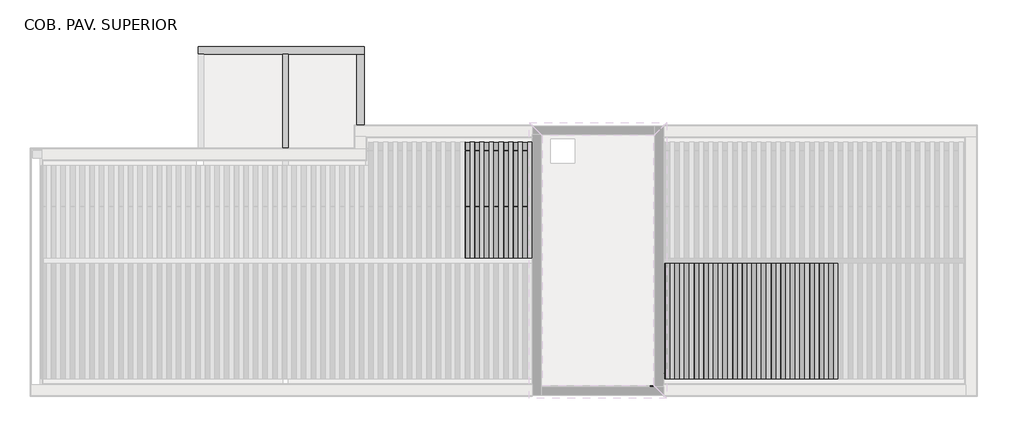
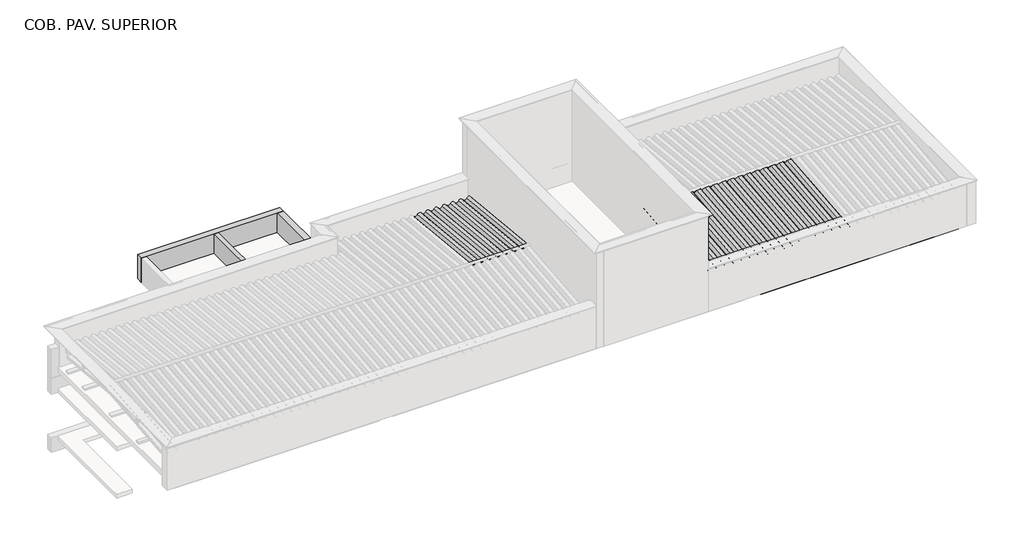
# One storey, part 5 of 7: 41 beams, 9 columns.
"""IFC4 building model written with IfcOpenShell, lengths in millimetres."""

import ifcopenshell
import ifcopenshell.guid

model = None  # the IFC model being written
_history = None  # IfcOwnerHistory: only IFC2X3 demands one
_inside = {}  # id of a spatial element -> (the spatial element, [elements in it])
_under = {}  # id of a project, library or spatial element -> (it, [spatial elements below it])
_declared = {}  # id of a project -> (the project, [libraries it declares])
_typed = {}  # id of a type object -> (the type object, [elements of that type])
_made_of = {}  # id of a material, layer set ... -> (it, [elements and type objects made of it])


def new_model(schema):
    """Start an empty IFC model of exactly this schema.

    Asked for "IFC4X3", IfcOpenShell would pick the latest addendum, in which some entities
    have other attributes; the version numbers below select the first issue.
    IFC2X3 requires an IfcOwnerHistory on every rooted entity: one is made here for all.
    """
    global model, _history
    if schema == "IFC4X3":
        model = ifcopenshell.file(schema_version=(4, 3, 0, 0))
    else:
        model = ifcopenshell.file(schema=schema)
    _inside.clear()
    _under.clear()
    _declared.clear()
    _typed.clear()
    _made_of.clear()
    _history = None
    if model.schema == "IFC2X3":
        org = make("IfcOrganization", Name="unknown")
        user = make(
            "IfcPersonAndOrganization",
            ThePerson=make("IfcPerson", FamilyName="unknown"),
            TheOrganization=org,
        )
        app = make(
            "IfcApplication",
            ApplicationDeveloper=org,
            Version="unknown",
            ApplicationFullName="unknown",
            ApplicationIdentifier="unknown",
        )
        _history = make(
            "IfcOwnerHistory",
            OwningUser=user,
            OwningApplication=app,
            ChangeAction="ADDED",
            CreationDate=0,
        )
    return model


def make(cls, **values):
    """One entity of the class cls with the attributes given. An attribute that is None is left unset."""
    return model.create_entity(
        cls, **{name: value for name, value in values.items() if value is not None}
    )


def rooted(cls, **values):
    """An entity with a GlobalId (a new one), such as an element, a storey or a relation."""
    return make(cls, GlobalId=ifcopenshell.guid.new(), OwnerHistory=_history, **values)


def si_unit(unit_type, name, prefix=None):
    """IfcSIUnit, for example si_unit("LENGTHUNIT", "METRE", prefix="MILLI")."""
    return make("IfcSIUnit", UnitType=unit_type, Prefix=prefix, Name=name)


def assignment(units):
    """IfcUnitAssignment: the units of a project."""
    return None if units is None else make("IfcUnitAssignment", Units=units)


def point(xyz):
    """IfcCartesianPoint."""
    return None if xyz is None else make("IfcCartesianPoint", Coordinates=xyz)


def direction(xyz):
    """IfcDirection."""
    return None if xyz is None else make("IfcDirection", DirectionRatios=xyz)


def frame(location, z_axis=None, x_axis=None):
    """IfcAxis2Placement3D, a coordinate frame: its origin and axes. An axis left out is left unset."""
    return make(
        "IfcAxis2Placement3D",
        Location=point(location),
        Axis=direction(z_axis),
        RefDirection=direction(x_axis),
    )


def frame_2d(location, x_axis=None):
    """IfcAxis2Placement2D, a coordinate frame in the plane: its origin and x axis."""
    return make(
        "IfcAxis2Placement2D", Location=point(location), RefDirection=direction(x_axis)
    )


def origin():
    """The frame at (0, 0, 0) with its axes left unset."""
    return frame((0.0, 0.0, 0.0))


def place(relative_to, where):
    """IfcLocalPlacement: puts the frame where relative to a parent placement (None: the world)."""
    return make(
        "IfcLocalPlacement", PlacementRelTo=relative_to, RelativePlacement=where
    )


def context(
    kind, dimensions, precision=None, world=None, true_north=None, identifier=None
):
    """IfcGeometricRepresentationContext, for example the 3D "Model" context."""
    return make(
        "IfcGeometricRepresentationContext",
        ContextIdentifier=identifier,
        ContextType=kind,
        CoordinateSpaceDimension=dimensions,
        Precision=precision,
        WorldCoordinateSystem=world,
        TrueNorth=true_north,
    )


def project(units=None, contexts=None):
    """IfcProject with its units and contexts."""
    return rooted(
        "IfcProject",
        Name="project",
        RepresentationContexts=contexts,
        UnitsInContext=assignment(units),
    )


def spatial(cls, under=None, at=None, **own):
    """A site, building, storey or space (cls), placed at a placement, below another one or the project."""
    s = rooted(cls, ObjectPlacement=at, **own)
    if under is not None:
        _under.setdefault(under.id(), (under, []))[1].append(s)
    return s


def polyline(points):
    """IfcPolyline through the points."""
    return make("IfcPolyline", Points=[point(p) for p in points])


def circle_curve(where, radius):
    """IfcCircle in the frame where."""
    return make("IfcCircle", Position=where, Radius=radius)


def trimmed(basis, trim1, trim2, sense, master):
    """IfcTrimmedCurve: the piece of a basis curve between two trims."""
    return make(
        "IfcTrimmedCurve",
        BasisCurve=basis,
        Trim1=trim1,
        Trim2=trim2,
        SenseAgreement=sense,
        MasterRepresentation=master,
    )


def segment(curve, same_sense, transition):
    """IfcCompositeCurveSegment."""
    return make(
        "IfcCompositeCurveSegment",
        Transition=transition,
        SameSense=same_sense,
        ParentCurve=curve,
    )


def composite_curve(segments, self_intersect=None):
    """IfcCompositeCurve: segments joined end to end."""
    return make("IfcCompositeCurve", Segments=segments, SelfIntersect=self_intersect)


def outline(outer, holes=None, kind="AREA"):
    """IfcArbitraryClosedProfileDef: a profile drawn as a closed curve; with holes, ...WithVoids."""
    if holes is None:
        return make("IfcArbitraryClosedProfileDef", ProfileType=kind, OuterCurve=outer)
    return make(
        "IfcArbitraryProfileDefWithVoids",
        ProfileType=kind,
        OuterCurve=outer,
        InnerCurves=holes,
    )


def extrude(swept, where, along, depth):
    """IfcExtrudedAreaSolid: the profile swept, set in the frame where, extruded along a direction by depth."""
    return make(
        "IfcExtrudedAreaSolid",
        SweptArea=swept,
        Position=where,
        ExtrudedDirection=direction(along),
        Depth=depth,
    )


def faces_of(points, faces, orient=None, outer=None):
    """IfcFace entities. A face is a list of loops; a loop is a list of indices into points, from 0.

    orient and outer hold one flag for each loop. By default every Orientation is true, the
    first loop of a face is its IfcFaceOuterBound and the others are IfcFaceBound.
    """
    made = []
    for i, loops in enumerate(faces):
        bounds = []
        for j, loop in enumerate(loops):
            is_outer = j == 0 if outer is None else outer[i][j]
            bounds.append(
                make(
                    "IfcFaceOuterBound" if is_outer else "IfcFaceBound",
                    Bound=make("IfcPolyLoop", Polygon=[points[k] for k in loop]),
                    Orientation=True if orient is None else orient[i][j],
                )
            )
        made.append(make("IfcFace", Bounds=bounds))
    return made


def faceted_brep(points, faces, orient=None, outer=None, voids=None):
    """IfcFacetedBrep: a solid bounded by flat faces; with voids (closed shells), ...WithVoids."""
    shared = [point(p) for p in points]
    hull = make("IfcClosedShell", CfsFaces=faces_of(shared, faces, orient, outer))
    if voids is None:
        return make("IfcFacetedBrep", Outer=hull)
    return make(
        "IfcFacetedBrepWithVoids",
        Outer=hull,
        Voids=[
            make(cls, CfsFaces=faces_of(shared, fs, o, b)) for cls, fs, o, b in voids
        ],
    )


def shape(context_of_items, identifier, shape_type, items):
    """IfcShapeRepresentation: the items that make up one representation, for example the "Body"."""
    return make(
        "IfcShapeRepresentation",
        ContextOfItems=context_of_items,
        RepresentationIdentifier=identifier,
        RepresentationType=shape_type,
        Items=items,
    )


def source(mapping_origin, context_of_items, identifier, shape_type, items):
    """IfcRepresentationMap: a shape defined once, which mapped items show again and again."""
    return make(
        "IfcRepresentationMap",
        MappingOrigin=mapping_origin,
        MappedRepresentation=shape(context_of_items, identifier, shape_type, items),
    )


def transform(
    local_origin,
    x_axis=None,
    y_axis=None,
    z_axis=None,
    scale=None,
    scale2=None,
    scale3=None,
    uniform=True,
):
    """IfcCartesianTransformationOperator3D, or its non-uniform kind. x_axis, y_axis, z_axis: its Axis1, 2, 3."""
    if uniform:
        return make(
            "IfcCartesianTransformationOperator3D",
            Axis1=direction(x_axis),
            Axis2=direction(y_axis),
            LocalOrigin=point(local_origin),
            Scale=scale,
            Axis3=direction(z_axis),
        )
    return make(
        "IfcCartesianTransformationOperator3DnonUniform",
        Axis1=direction(x_axis),
        Axis2=direction(y_axis),
        LocalOrigin=point(local_origin),
        Scale=scale,
        Axis3=direction(z_axis),
        Scale2=scale2,
        Scale3=scale3,
    )


def mapped(mapping_source, mapping_target):
    """IfcMappedItem: shows the shape of a source again, moved by a transform."""
    return make(
        "IfcMappedItem", MappingSource=mapping_source, MappingTarget=mapping_target
    )


def made_of(thing, what):
    """Note that an element or type object is made of a material, layer set ...; save() writes the relation."""
    if what is not None:
        _made_of.setdefault(what.id(), (what, []))[1].append(thing)
    return thing


def element(
    cls,
    number,
    at=None,
    inside=None,
    cuts=None,
    type_object=None,
    material=None,
    context=None,
    identifier="Body",
    shape_type=None,
    held_by="IfcProductDefinitionShape",
    body=None,
    shapes=None,
    **own,
):
    """One element of the class cls, such as IfcWall. Its Tag is "e" and its number.

    at: its placement. inside: the storey or other place that contains it. cuts: it is an
    opening in that element (IfcRelVoidsElement). A single representation is given by context,
    identifier, shape_type and body (its items); several are given by shapes. held_by: the class
    of the entity that holds the representations. save() writes the other relations.
    """
    e = rooted(cls, Tag="e%d" % number, ObjectPlacement=at, **own)
    if body is not None:
        shapes = [shape(context, identifier, shape_type, body)]
    if shapes is not None:
        e.Representation = make(held_by, Representations=shapes)
    if inside is not None:
        _inside.setdefault(inside.id(), (inside, []))[1].append(e)
    if cuts is not None:
        rooted(
            "IfcRelVoidsElement", RelatingBuildingElement=cuts, RelatedOpeningElement=e
        )
    if type_object is not None:
        _typed.setdefault(type_object.id(), (type_object, []))[1].append(e)
    return made_of(e, material)


def aggregate(whole, parts):
    """IfcRelAggregates: a whole, such as a stair, and the parts it consists of."""
    return rooted("IfcRelAggregates", RelatingObject=whole, RelatedObjects=parts)


def save(model, path):
    """Write the relations noted so far, then the file.

    IfcRelAggregates (storeys below a building ...), IfcRelContainedInSpatialStructure (elements
    in a storey), IfcRelDefinesByType, IfcRelAssociatesMaterial and IfcRelDeclares: one each for
    every whole, place, type object, material and project.
    """
    for whole, parts in _under.values():
        aggregate(whole, parts)
    for where, things in _inside.values():
        rooted(
            "IfcRelContainedInSpatialStructure",
            RelatedElements=things,
            RelatingStructure=where,
        )
    for kind, things in _typed.values():
        rooted("IfcRelDefinesByType", RelatedObjects=things, RelatingType=kind)
    for what, things in _made_of.values():
        rooted("IfcRelAssociatesMaterial", RelatedObjects=things, RelatingMaterial=what)
    for by, libraries in _declared.values():
        rooted("IfcRelDeclares", RelatingContext=by, RelatedDefinitions=libraries)
    model.write(path)


def column_d505325c(model_context):
    return source(origin(), model_context, "Body", "SweptSolid", [
        extrude(outline(polyline([(30.0, 80.0), (30.0, -80.0), (-30.0, -80.0), (-30.0, 80.0), (30.0, 80.0)])), frame((0.0, 0.0, 6710.0), z_axis=(0.0, 0.0, 1.0), x_axis=(1.0, 0.0, 0.0)), (0.0, 0.0, 1.0), 750.0),
    ])


def column_4db371bd(model_context):
    return source(origin(), model_context, "Body", "SweptSolid", [
        extrude(outline(polyline([(30.0, 80.0), (30.0, -80.0), (-30.0, -80.0), (-30.0, 80.0), (30.0, 80.0)])), frame((0.0, 0.0, 6710.0), z_axis=(0.0, 0.0, 1.0), x_axis=(1.0, 0.0, 0.0)), (0.0, 0.0, 1.0), 660.0),
    ])


def column_e8b88e91(model_context):
    return source(origin(), model_context, "Body", "SweptSolid", [
        extrude(outline(polyline([(30.0, 80.0), (30.0, -80.0), (-30.0, -80.0), (-30.0, 80.0), (30.0, 80.0)])), frame((0.0, 0.0, 6710.0), z_axis=(0.0, 0.0, 1.0), x_axis=(1.0, 0.0, 0.0)), (0.0, 0.0, 1.0), 515.0),
    ])


def column_d0cf395a(model_context):
    return source(origin(), model_context, "Body", "SweptSolid", [
        extrude(outline(polyline([(30.0, 80.0), (30.0, -80.0), (-30.0, -80.0), (-30.0, 80.0), (30.0, 80.0)])), frame((0.0, 0.0, 6710.0), z_axis=(0.0, 0.0, 1.0), x_axis=(1.0, 0.0, 0.0)), (0.0, 0.0, 1.0), 520.0),
    ])


model = new_model("IFC4")

# Units and contexts
model_context = context("Model", 3, world=origin())
ifc_project = project(units=[si_unit("LENGTHUNIT", "METRE", prefix="MILLI")], contexts=[model_context])

# Site, building, storey
site = spatial("IfcSite", under=ifc_project)
building = spatial("IfcBuilding", under=site)
storey = spatial("IfcBuildingStorey", under=building, Name="COB. PAV. SUPERIOR", Elevation=6650.0)

# Beams
placement = place(None, origin())
element("IfcBeam", 1, ObjectType="Madeira de lei : Berço 6x12cm", at=placement, inside=storey, context=model_context, shape_type="SweptSolid", body=[
    extrude(outline(polyline([(-679.281307, -7711.5607799), (-679.281307, -7831.5607799), (-2679.281307, -7831.5607799), (-2679.281307, -7711.5607799), (-679.281307, -7711.5607799)])), frame((0.0, 0.0, 6650.0), z_axis=(0.0, 0.0, 1.0), x_axis=(1.0, 0.0, 0.0)), (0.0, 0.0, 1.0), 60.0),
])
element("IfcBeam", 2, ObjectType="Madeira de lei : Berço 6x12cm", at=placement, inside=storey, context=model_context, shape_type="SweptSolid", body=[
    extrude(outline(polyline([(-244.281307, -7711.5607799), (-244.281307, -7831.5607799), (-679.281307, -7831.5607799), (-679.281307, -7711.5607799), (-244.281307, -7711.5607799)])), frame((0.0, 0.0, 6650.0), z_axis=(0.0, 0.0, 1.0), x_axis=(1.0, 0.0, 0.0)), (0.0, 0.0, 1.0), 60.0),
])
element("IfcBeam", 3, ObjectType="Madeira de lei : Berço 6x12cm", at=placement, inside=storey, context=model_context, shape_type="SweptSolid", body=[
    extrude(outline(polyline([(-679.2813076, -6319.8711004), (-679.2813076, -6439.8711004), (-2679.2813064, -6439.8711004), (-2679.2813064, -6319.8711004), (-679.2813076, -6319.8711004)])), frame((0.0, 0.0, 6650.0), z_axis=(0.0, 0.0, 1.0), x_axis=(1.0, 0.0, 0.0)), (0.0, 0.0, 1.0), 60.0),
])
element("IfcBeam", 4, ObjectType="Madeira de lei : Berço 6x12cm", at=placement, inside=storey, context=model_context, shape_type="SweptSolid", body=[
    extrude(outline(polyline([(-259.281307, -6319.8711004), (-259.281307, -6439.8711004), (-679.2813064, -6439.8711004), (-679.2813064, -6319.8711004), (-259.281307, -6319.8711004)])), frame((0.0, 0.0, 6650.0), z_axis=(0.0, 0.0, 1.0), x_axis=(1.0, 0.0, 0.0)), (0.0, 0.0, 1.0), 60.0),
])
element("IfcBeam", 5, ObjectType="Madeira de lei : Berço 6x12cm", at=placement, inside=storey, context=model_context, shape_type="SweptSolid", body=[
    extrude(outline(polyline([(5089.718693, -9101.268869), (5089.718693, -9221.268869), (3089.718693, -9221.268869), (3089.718693, -9101.268869), (5089.718693, -9101.268869)])), frame((0.0, 0.0, 6650.0), z_axis=(0.0, 0.0, 1.0), x_axis=(1.0, 0.0, 0.0)), (0.0, 0.0, 1.0), 60.0),
])
element("IfcBeam", 6, ObjectType="Madeira de lei : Berço 6x12cm", at=placement, inside=storey, context=model_context, shape_type="SweptSolid", body=[
    extrude(outline(polyline([(5089.718693, -10521.818869), (5089.718693, -10641.818869), (3089.718693, -10641.818869), (3089.718693, -10521.818869), (5089.718693, -10521.818869)])), frame((0.0, 0.0, 6650.0), z_axis=(0.0, 0.0, 1.0), x_axis=(1.0, 0.0, 0.0)), (0.0, 0.0, 1.0), 60.0),
])
element("IfcBeam", 7, ObjectType="Madeira de lei : Berço 6x12cm", at=placement, inside=storey, context=model_context, shape_type="SweptSolid", body=[
    extrude(outline(polyline([(7089.718693, -9101.268869), (7089.718693, -9221.268869), (5089.718693, -9221.268869), (5089.718693, -9101.268869), (7089.718693, -9101.268869)])), frame((0.0, 0.0, 6650.0), z_axis=(0.0, 0.0, 1.0), x_axis=(1.0, 0.0, 0.0)), (0.0, 0.0, 1.0), 60.0),
])
element("IfcBeam", 8, ObjectType="Madeira de lei : Berço 6x12cm", at=placement, inside=storey, context=model_context, shape_type="SweptSolid", body=[
    extrude(outline(polyline([(7089.718693, -10521.818869), (7089.718693, -10641.818869), (5089.718693, -10641.818869), (5089.718693, -10521.818869), (7089.718693, -10521.818869)])), frame((0.0, 0.0, 6650.0), z_axis=(0.0, 0.0, 1.0), x_axis=(1.0, 0.0, 0.0)), (0.0, 0.0, 1.0), 60.0),
])
element("IfcBeam", 9, ObjectType="Madeira de lei : Berço 6x12cm", at=placement, inside=storey, context=model_context, shape_type="SweptSolid", body=[
    extrude(outline(polyline([(-270.281307, -4899.3026908), (-270.281307, -5019.3026908), (-2270.2813064, -5019.3026908), (-2270.2813064, -4899.3026908), (-270.281307, -4899.3026908)])), frame((0.0, 0.0, 6650.0), z_axis=(0.0, 0.0, 1.0), x_axis=(1.0, 0.0, 0.0)), (0.0, 0.0, 1.0), 60.0),
])
element("IfcBeam", 10, ObjectType="Madeira de lei : Berço 6x12cm", at=placement, inside=storey, context=model_context, shape_type="SweptSolid", body=[
    extrude(outline(polyline([(-2270.2813076, -4899.3026908), (-2270.2813076, -5019.3026908), (-4270.281307, -5019.3026908), (-4270.281307, -4899.3026908), (-2270.2813076, -4899.3026908)])), frame((0.0, 0.0, 6650.0), z_axis=(0.0, 0.0, 1.0), x_axis=(1.0, 0.0, 0.0)), (0.0, 0.0, 1.0), 60.0),
])
element("IfcBeam", 11, ObjectType="TQS - Viga retangular : 14.0 x 76.0", at=placement, inside=storey, context=model_context, shape_type="Brep", body=[
    faceted_brep([(-6580.281307, -4975.5699847, 7050.0), (-6440.281307, -4975.5699847, 7050.0), (-6440.281307, -2515.5699847, 7050.0), (-6580.281307, -2515.5699847, 7050.0), (-6440.281307, -4975.5699847, 6450.0), (-6440.281307, -4975.5699847, 6290.0), (-6440.281307, -2515.5699847, 6290.0), (-6440.281307, -2515.5699847, 6450.0), (-6580.281307, -4975.5699847, 6290.0), (-6580.281307, -2515.5699847, 6290.0), (-6580.281307, -4975.5699847, 6450.0), (-6580.281307, -2515.5699847, 6450.0)], [[[0, 1, 2, 3]], [[1, 4, 5, 6, 7, 2]], [[5, 8, 9, 6]], [[8, 10, 0, 3, 11, 9]], [[0, 10, 8, 5, 4, 1]], [[3, 2, 7, 6, 9, 11]]]),
])
element("IfcBeam", 12, ObjectType="TQS - Viga retangular : 19.0 x 60.0", at=placement, inside=storey, context=model_context, shape_type="Brep", body=[
    faceted_brep([(-12.281307, -4775.5699847, 7050.0), (-202.281307, -4775.5699847, 7050.0), (-202.281307, -10953.5699847, 7050.0), (-12.281307, -10953.5699847, 7050.0), (-12.281307, -4775.5699847, 6450.0), (-12.281307, -10953.5699847, 6650.0), (-12.281307, -10953.5699847, 6450.0), (-202.281307, -4775.5699847, 6450.0), (-202.281307, -10953.5699847, 6450.0), (-202.281307, -10953.5699847, 6650.0)], [[[0, 1, 2, 3]], [[4, 0, 3, 5, 6]], [[7, 4, 6, 8]], [[1, 7, 8, 9, 2]], [[1, 0, 4, 7]], [[2, 9, 8, 6, 5, 3]]]),
])
element("IfcBeam", 13, ObjectType="TQS - Viga retangular : 19.0 x 76.0", at=placement, inside=storey, context=model_context, shape_type="Brep", body=[
    faceted_brep([(-8730.281307, -2325.5699847, 7050.0), (-8730.281307, -2515.5699847, 7050.0), (-8590.281307, -2515.5699847, 7050.0), (-6580.281307, -2515.5699847, 7050.0), (-6440.281307, -2515.5699847, 7050.0), (-4702.281307, -2515.5699847, 7050.0), (-4512.281307, -2515.5699847, 7050.0), (-4512.281307, -2325.5699847, 7050.0), (-8730.281307, -2515.5699847, 6290.0), (-8590.281307, -2515.5699847, 6290.0), (-6580.281307, -2515.5699847, 6290.0), (-6440.281307, -2515.5699847, 6290.0), (-4702.281307, -2515.5699847, 6290.0), (-4512.281307, -2515.5699847, 6290.0), (-8730.281307, -2325.5699847, 6290.0), (-4512.281307, -2325.5699847, 6290.0)], [[[0, 1, 2, 3, 4, 5, 6, 7]], [[1, 8, 9, 10, 11, 12, 13, 6, 5, 4, 3, 2]], [[8, 14, 15, 13, 12, 11, 10, 9]], [[14, 0, 7, 15]], [[1, 0, 14, 8]], [[7, 6, 13, 15]]]),
])
element("IfcBeam", 14, ObjectType="TQS - Viga retangular : 19.0 x 76.0", at=placement, inside=storey, context=model_context, shape_type="Brep", body=[
    faceted_brep([(-4512.281307, -2515.5699847, 7050.0), (-4702.281307, -2515.5699847, 7050.0), (-4702.281307, -4375.5699847, 7050.0), (-4512.281307, -4375.5699847, 7050.0), (-4512.281307, -2515.5699847, 6290.0), (-4512.281307, -4375.5699847, 6290.0), (-4702.281307, -2515.5699847, 6290.0), (-4702.281307, -4375.5699847, 6290.0), (-4702.281307, -2515.5699847, 6450.0)], [[[0, 1, 2, 3]], [[4, 0, 3, 5]], [[6, 4, 5, 7]], [[1, 8, 6, 7, 2]], [[1, 0, 4, 6, 8]], [[3, 2, 7, 5]]]),
])
element("IfcBeam", 15, ObjectType="TQS - Viga retangular : 19.0 x 80.0", at=placement, inside=storey, context=model_context, shape_type="SweptSolid", body=[
    extrude(outline(polyline([(10537.718693, -10953.5699847), (10537.718693, -11143.5699847), (4678.718693, -11143.5699847), (4678.718693, -10953.5699847), (10537.718693, -10953.5699847)])), frame((0.0, 0.0, 6450.0), z_axis=(0.0, 0.0, 1.0), x_axis=(1.0, 0.0, 0.0)), (0.0, 0.0, 1.0), 800.0),
])
element("IfcBeam", 16, ObjectType="TQS - Viga retangular : 19.0 x 80.0", at=placement, inside=storey, context=model_context, shape_type="Brep", body=[
    faceted_brep([(-4142.481307, -4375.5699847, 7250.0), (-4142.481307, -4565.5699847, 7250.0), (-202.281307, -4565.5699847, 7250.0), (-202.281307, -4375.5699847, 7250.0), (-4142.481307, -4565.5699847, 6450.0), (-202.281307, -4565.5699847, 6450.0), (-202.281307, -4565.5699847, 6650.0), (-4142.481307, -4375.5699847, 6450.0), (-202.281307, -4375.5699847, 6450.0)], [[[0, 1, 2, 3]], [[1, 4, 5, 6, 2]], [[4, 7, 8, 5]], [[7, 0, 3, 8]], [[1, 0, 7, 4]], [[3, 2, 6, 5, 8]]]),
    faceted_brep([(-4442.481307, -4375.5699847, 7250.0), (-4442.481307, -4565.5699847, 7250.0), (-4442.481307, -4565.5699847, 6450.0), (-4442.481307, -4375.5699847, 6450.0), (-4512.281307, -4375.5699847, 7250.0), (-4512.281307, -4565.5699847, 7250.0), (-4512.281307, -4565.5699847, 6650.0), (-4512.281307, -4565.5699847, 6450.0), (-4512.281307, -4375.5699847, 6450.0)], [[[0, 1, 2, 3]], [[1, 0, 4, 5]], [[2, 1, 5, 6, 7]], [[3, 2, 7, 8]], [[0, 3, 8, 4]], [[5, 4, 8, 7, 6]]]),
])
element("IfcBeam", 17, ObjectType="Telha Ondulada : Fibrocimento", at=placement, inside=storey, context=model_context, shape_type="SweptSolid", body=[
    extrude(outline(composite_curve([segment(trimmed(circle_curve(frame_2d((0.0, 66.7939461)), 66.7939461), [point((29.3501489, 6.7939461))], [point((29.3501489, 126.7939461))], True, "CARTESIAN"), True, "CONTINUOUS"), segment(polyline([(29.3501489, 126.7939461), (31.5472154, 131.2853711)]), True, "CONTINUOUS"), segment(trimmed(circle_curve(frame_2d((0.0, 66.7939461)), 71.7939461), [point((31.5472154, 131.2853711))], [point((31.5472154, 2.3025211))], False, "CARTESIAN"), True, "CONTINUOUS"), segment(trimmed(circle_curve(frame_2d((58.7002978, -53.2060539)), 61.7939461), [point((31.5472154, 2.3025211))], [point((31.5472154, -108.7146289))], True, "CARTESIAN"), True, "CONTINUOUS"), segment(polyline([(31.5472154, -108.7146289), (29.3501489, -113.2060539)]), True, "CONTINUOUS"), segment(trimmed(circle_curve(frame_2d((58.7002978, -53.2060539)), 66.7939461), [point((29.3501489, -113.2060539))], [point((29.3501489, 6.7939461))], False, "CARTESIAN"), True, "CONTINUOUS")], self_intersect=False)), frame((3256.1156257, -10781.9594023, 7394.5315886), z_axis=(0.0, 0.9950371902099894, 0.09950371902099751), x_axis=(0.0, 0.09950371902099751, -0.9950371902099894)), (0.0, 0.0, 1.0), 3017.2387654),
])
element("IfcBeam", 18, ObjectType="Telha Ondulada : Fibrocimento", at=placement, inside=storey, context=model_context, shape_type="SweptSolid", body=[
    extrude(outline(composite_curve([segment(trimmed(circle_curve(frame_2d((0.0, 66.7939461)), 66.7939461), [point((29.3501489, 6.7939461))], [point((29.3501489, 126.7939461))], True, "CARTESIAN"), True, "CONTINUOUS"), segment(polyline([(29.3501489, 126.7939461), (31.5472154, 131.2853711)]), True, "CONTINUOUS"), segment(trimmed(circle_curve(frame_2d((0.0, 66.7939461)), 71.7939461), [point((31.5472154, 131.2853711))], [point((31.5472154, 2.3025211))], False, "CARTESIAN"), True, "CONTINUOUS"), segment(trimmed(circle_curve(frame_2d((58.7002978, -53.2060539)), 61.7939461), [point((31.5472154, 2.3025211))], [point((31.5472154, -108.7146289))], True, "CARTESIAN"), True, "CONTINUOUS"), segment(polyline([(31.5472154, -108.7146289), (29.3501489, -113.2060539)]), True, "CONTINUOUS"), segment(trimmed(circle_curve(frame_2d((58.7002978, -53.2060539)), 66.7939461), [point((29.3501489, -113.2060539))], [point((29.3501489, 6.7939461))], False, "CARTESIAN"), True, "CONTINUOUS")], self_intersect=False)), frame((3500.6156257, -10781.9594023, 7394.5315886), z_axis=(0.0, 0.9950371902099894, 0.09950371902099751), x_axis=(0.0, 0.09950371902099751, -0.9950371902099894)), (0.0, 0.0, 1.0), 3017.2387654),
])
element("IfcBeam", 19, ObjectType="Telha Ondulada : Fibrocimento", at=placement, inside=storey, context=model_context, shape_type="SweptSolid", body=[
    extrude(outline(composite_curve([segment(trimmed(circle_curve(frame_2d((0.0, 66.7939461)), 66.7939461), [point((29.3501489, 6.7939461))], [point((29.3501489, 126.7939461))], True, "CARTESIAN"), True, "CONTINUOUS"), segment(polyline([(29.3501489, 126.7939461), (31.5472154, 131.2853711)]), True, "CONTINUOUS"), segment(trimmed(circle_curve(frame_2d((0.0, 66.7939461)), 71.7939461), [point((31.5472154, 131.2853711))], [point((31.5472154, 2.3025211))], False, "CARTESIAN"), True, "CONTINUOUS"), segment(trimmed(circle_curve(frame_2d((58.7002978, -53.2060539)), 61.7939461), [point((31.5472154, 2.3025211))], [point((31.5472154, -108.7146289))], True, "CARTESIAN"), True, "CONTINUOUS"), segment(polyline([(31.5472154, -108.7146289), (29.3501489, -113.2060539)]), True, "CONTINUOUS"), segment(trimmed(circle_curve(frame_2d((58.7002978, -53.2060539)), 66.7939461), [point((29.3501489, -113.2060539))], [point((29.3501489, 6.7939461))], False, "CARTESIAN"), True, "CONTINUOUS")], self_intersect=False)), frame((3745.1156257, -10781.9594023, 7394.5315886), z_axis=(0.0, 0.9950371902099894, 0.09950371902099751), x_axis=(0.0, 0.09950371902099751, -0.9950371902099894)), (0.0, 0.0, 1.0), 3017.2387654),
])
element("IfcBeam", 20, ObjectType="Telha Ondulada : Fibrocimento", at=placement, inside=storey, context=model_context, shape_type="SweptSolid", body=[
    extrude(outline(composite_curve([segment(trimmed(circle_curve(frame_2d((0.0, 66.7939461)), 66.7939461), [point((29.3501489, 6.7939461))], [point((29.3501489, 126.7939461))], True, "CARTESIAN"), True, "CONTINUOUS"), segment(polyline([(29.3501489, 126.7939461), (31.5472154, 131.2853711)]), True, "CONTINUOUS"), segment(trimmed(circle_curve(frame_2d((0.0, 66.7939461)), 71.7939461), [point((31.5472154, 131.2853711))], [point((31.5472154, 2.3025211))], False, "CARTESIAN"), True, "CONTINUOUS"), segment(trimmed(circle_curve(frame_2d((58.7002978, -53.2060539)), 61.7939461), [point((31.5472154, 2.3025211))], [point((31.5472154, -108.7146289))], True, "CARTESIAN"), True, "CONTINUOUS"), segment(polyline([(31.5472154, -108.7146289), (29.3501489, -113.2060539)]), True, "CONTINUOUS"), segment(trimmed(circle_curve(frame_2d((58.7002978, -53.2060539)), 66.7939461), [point((29.3501489, -113.2060539))], [point((29.3501489, 6.7939461))], False, "CARTESIAN"), True, "CONTINUOUS")], self_intersect=False)), frame((3989.6156257, -10781.9594023, 7394.5315886), z_axis=(0.0, 0.9950371902099894, 0.09950371902099747), x_axis=(0.0, 0.09950371902099747, -0.9950371902099894)), (0.0, 0.0, 1.0), 3017.2387654),
])
element("IfcBeam", 21, ObjectType="Telha Ondulada : Fibrocimento", at=placement, inside=storey, context=model_context, shape_type="SweptSolid", body=[
    extrude(outline(composite_curve([segment(trimmed(circle_curve(frame_2d((0.0, 66.7939461)), 66.7939461), [point((29.3501489, 6.7939461))], [point((29.3501489, 126.7939461))], True, "CARTESIAN"), True, "CONTINUOUS"), segment(polyline([(29.3501489, 126.7939461), (31.5472154, 131.2853711)]), True, "CONTINUOUS"), segment(trimmed(circle_curve(frame_2d((0.0, 66.7939461)), 71.7939461), [point((31.5472154, 131.2853711))], [point((31.5472154, 2.3025211))], False, "CARTESIAN"), True, "CONTINUOUS"), segment(trimmed(circle_curve(frame_2d((58.7002978, -53.2060539)), 61.7939461), [point((31.5472154, 2.3025211))], [point((31.5472154, -108.7146289))], True, "CARTESIAN"), True, "CONTINUOUS"), segment(polyline([(31.5472154, -108.7146289), (29.3501489, -113.2060539)]), True, "CONTINUOUS"), segment(trimmed(circle_curve(frame_2d((58.7002978, -53.2060539)), 66.7939461), [point((29.3501489, -113.2060539))], [point((29.3501489, 6.7939461))], False, "CARTESIAN"), True, "CONTINUOUS")], self_intersect=False)), frame((4234.1156257, -10781.9594023, 7394.5315886), z_axis=(0.0, 0.9950371902099894, 0.09950371902099747), x_axis=(0.0, 0.09950371902099747, -0.9950371902099894)), (0.0, 0.0, 1.0), 3017.2387654),
])
element("IfcBeam", 22, ObjectType="Telha Ondulada : Fibrocimento", at=placement, inside=storey, context=model_context, shape_type="SweptSolid", body=[
    extrude(outline(composite_curve([segment(trimmed(circle_curve(frame_2d((0.0, 66.7939461)), 66.7939461), [point((29.3501489, 6.7939461))], [point((29.3501489, 126.7939461))], True, "CARTESIAN"), True, "CONTINUOUS"), segment(polyline([(29.3501489, 126.7939461), (31.5472154, 131.2853711)]), True, "CONTINUOUS"), segment(trimmed(circle_curve(frame_2d((0.0, 66.7939461)), 71.7939461), [point((31.5472154, 131.2853711))], [point((31.5472154, 2.3025211))], False, "CARTESIAN"), True, "CONTINUOUS"), segment(trimmed(circle_curve(frame_2d((58.7002978, -53.2060539)), 61.7939461), [point((31.5472154, 2.3025211))], [point((31.5472154, -108.7146289))], True, "CARTESIAN"), True, "CONTINUOUS"), segment(polyline([(31.5472154, -108.7146289), (29.3501489, -113.2060539)]), True, "CONTINUOUS"), segment(trimmed(circle_curve(frame_2d((58.7002978, -53.2060539)), 66.7939461), [point((29.3501489, -113.2060539))], [point((29.3501489, 6.7939461))], False, "CARTESIAN"), True, "CONTINUOUS")], self_intersect=False)), frame((4478.6156257, -10781.9594023, 7394.5315886), z_axis=(0.0, 0.9950371902099894, 0.09950371902099744), x_axis=(0.0, 0.09950371902099744, -0.9950371902099894)), (0.0, 0.0, 1.0), 3017.2387654),
])
element("IfcBeam", 23, ObjectType="Telha Ondulada : Fibrocimento", at=placement, inside=storey, context=model_context, shape_type="SweptSolid", body=[
    extrude(outline(composite_curve([segment(trimmed(circle_curve(frame_2d((0.0, 66.7939461)), 66.7939461), [point((29.3501489, 6.7939461))], [point((29.3501489, 126.7939461))], True, "CARTESIAN"), True, "CONTINUOUS"), segment(polyline([(29.3501489, 126.7939461), (31.5472154, 131.2853711)]), True, "CONTINUOUS"), segment(trimmed(circle_curve(frame_2d((0.0, 66.7939461)), 71.7939461), [point((31.5472154, 131.2853711))], [point((31.5472154, 2.3025211))], False, "CARTESIAN"), True, "CONTINUOUS"), segment(trimmed(circle_curve(frame_2d((58.7002978, -53.2060539)), 61.7939461), [point((31.5472154, 2.3025211))], [point((31.5472154, -108.7146289))], True, "CARTESIAN"), True, "CONTINUOUS"), segment(polyline([(31.5472154, -108.7146289), (29.3501489, -113.2060539)]), True, "CONTINUOUS"), segment(trimmed(circle_curve(frame_2d((58.7002978, -53.2060539)), 66.7939461), [point((29.3501489, -113.2060539))], [point((29.3501489, 6.7939461))], False, "CARTESIAN"), True, "CONTINUOUS")], self_intersect=False)), frame((4723.1156257, -10781.9594023, 7394.5315886), z_axis=(0.0, 0.9950371902099894, 0.09950371902099751), x_axis=(0.0, 0.09950371902099751, -0.9950371902099894)), (0.0, 0.0, 1.0), 3017.2387654),
])
element("IfcBeam", 24, ObjectType="Telha Ondulada : Fibrocimento", at=placement, inside=storey, context=model_context, shape_type="SweptSolid", body=[
    extrude(outline(composite_curve([segment(trimmed(circle_curve(frame_2d((0.0, 66.7939461)), 66.7939461), [point((29.3501489, 6.7939461))], [point((29.3501489, 126.7939461))], True, "CARTESIAN"), True, "CONTINUOUS"), segment(polyline([(29.3501489, 126.7939461), (31.5472154, 131.2853711)]), True, "CONTINUOUS"), segment(trimmed(circle_curve(frame_2d((0.0, 66.7939461)), 71.7939461), [point((31.5472154, 131.2853711))], [point((31.5472154, 2.3025211))], False, "CARTESIAN"), True, "CONTINUOUS"), segment(trimmed(circle_curve(frame_2d((58.7002978, -53.2060539)), 61.7939461), [point((31.5472154, 2.3025211))], [point((31.5472154, -108.7146289))], True, "CARTESIAN"), True, "CONTINUOUS"), segment(polyline([(31.5472154, -108.7146289), (29.3501489, -113.2060539)]), True, "CONTINUOUS"), segment(trimmed(circle_curve(frame_2d((58.7002978, -53.2060539)), 66.7939461), [point((29.3501489, -113.2060539))], [point((29.3501489, 6.7939461))], False, "CARTESIAN"), True, "CONTINUOUS")], self_intersect=False)), frame((4967.6156257, -10781.9594023, 7394.5315886), z_axis=(0.0, 0.9950371902099894, 0.09950371902099751), x_axis=(0.0, 0.09950371902099751, -0.9950371902099894)), (0.0, 0.0, 1.0), 3017.2387654),
])
element("IfcBeam", 25, ObjectType="Telha Ondulada : Fibrocimento", at=placement, inside=storey, context=model_context, shape_type="SweptSolid", body=[
    extrude(outline(composite_curve([segment(trimmed(circle_curve(frame_2d((0.0, 66.7939461)), 66.7939461), [point((29.3501489, 6.7939461))], [point((29.3501489, 126.7939461))], True, "CARTESIAN"), True, "CONTINUOUS"), segment(polyline([(29.3501489, 126.7939461), (31.5472154, 131.2853711)]), True, "CONTINUOUS"), segment(trimmed(circle_curve(frame_2d((0.0, 66.7939461)), 71.7939461), [point((31.5472154, 131.2853711))], [point((31.5472154, 2.3025211))], False, "CARTESIAN"), True, "CONTINUOUS"), segment(trimmed(circle_curve(frame_2d((58.7002978, -53.2060539)), 61.7939461), [point((31.5472154, 2.3025211))], [point((31.5472154, -108.7146289))], True, "CARTESIAN"), True, "CONTINUOUS"), segment(polyline([(31.5472154, -108.7146289), (29.3501489, -113.2060539)]), True, "CONTINUOUS"), segment(trimmed(circle_curve(frame_2d((58.7002978, -53.2060539)), 66.7939461), [point((29.3501489, -113.2060539))], [point((29.3501489, 6.7939461))], False, "CARTESIAN"), True, "CONTINUOUS")], self_intersect=False)), frame((5212.1156257, -10781.9594023, 7394.5315886), z_axis=(0.0, 0.9950371902099894, 0.09950371902099751), x_axis=(0.0, 0.09950371902099751, -0.9950371902099894)), (0.0, 0.0, 1.0), 3017.2387654),
])
element("IfcBeam", 26, ObjectType="Telha Ondulada : Fibrocimento", at=placement, inside=storey, context=model_context, shape_type="SweptSolid", body=[
    extrude(outline(composite_curve([segment(trimmed(circle_curve(frame_2d((0.0, 66.7939461)), 66.7939461), [point((29.3501489, 6.7939461))], [point((29.3501489, 126.7939461))], True, "CARTESIAN"), True, "CONTINUOUS"), segment(polyline([(29.3501489, 126.7939461), (31.5472154, 131.2853711)]), True, "CONTINUOUS"), segment(trimmed(circle_curve(frame_2d((0.0, 66.7939461)), 71.7939461), [point((31.5472154, 131.2853711))], [point((31.5472154, 2.3025211))], False, "CARTESIAN"), True, "CONTINUOUS"), segment(trimmed(circle_curve(frame_2d((58.7002978, -53.2060539)), 61.7939461), [point((31.5472154, 2.3025211))], [point((31.5472154, -108.7146289))], True, "CARTESIAN"), True, "CONTINUOUS"), segment(polyline([(31.5472154, -108.7146289), (29.3501489, -113.2060539)]), True, "CONTINUOUS"), segment(trimmed(circle_curve(frame_2d((58.7002978, -53.2060539)), 66.7939461), [point((29.3501489, -113.2060539))], [point((29.3501489, 6.7939461))], False, "CARTESIAN"), True, "CONTINUOUS")], self_intersect=False)), frame((5456.6156257, -10781.9594023, 7394.5315886), z_axis=(0.0, 0.9950371902099894, 0.09950371902099751), x_axis=(0.0, 0.09950371902099751, -0.9950371902099894)), (0.0, 0.0, 1.0), 3017.2387654),
])
element("IfcBeam", 27, ObjectType="Telha Ondulada : Fibrocimento", at=placement, inside=storey, context=model_context, shape_type="SweptSolid", body=[
    extrude(outline(composite_curve([segment(trimmed(circle_curve(frame_2d((0.0, 66.7939461)), 66.7939461), [point((29.3501489, 6.7939461))], [point((29.3501489, 126.7939461))], True, "CARTESIAN"), True, "CONTINUOUS"), segment(polyline([(29.3501489, 126.7939461), (31.5472154, 131.2853711)]), True, "CONTINUOUS"), segment(trimmed(circle_curve(frame_2d((0.0, 66.7939461)), 71.7939461), [point((31.5472154, 131.2853711))], [point((31.5472154, 2.3025211))], False, "CARTESIAN"), True, "CONTINUOUS"), segment(trimmed(circle_curve(frame_2d((58.7002978, -53.2060539)), 61.7939461), [point((31.5472154, 2.3025211))], [point((31.5472154, -108.7146289))], True, "CARTESIAN"), True, "CONTINUOUS"), segment(polyline([(31.5472154, -108.7146289), (29.3501489, -113.2060539)]), True, "CONTINUOUS"), segment(trimmed(circle_curve(frame_2d((58.7002978, -53.2060539)), 66.7939461), [point((29.3501489, -113.2060539))], [point((29.3501489, 6.7939461))], False, "CARTESIAN"), True, "CONTINUOUS")], self_intersect=False)), frame((5701.1156257, -10781.9594023, 7394.5315886), z_axis=(0.0, 0.9950371902099894, 0.09950371902099747), x_axis=(0.0, 0.09950371902099747, -0.9950371902099894)), (0.0, 0.0, 1.0), 3017.2387654),
])
element("IfcBeam", 28, ObjectType="Telha Ondulada : Fibrocimento", at=placement, inside=storey, context=model_context, shape_type="SweptSolid", body=[
    extrude(outline(composite_curve([segment(trimmed(circle_curve(frame_2d((0.0, 66.7939461)), 66.7939461), [point((29.3501489, 6.7939461))], [point((29.3501489, 126.7939461))], True, "CARTESIAN"), True, "CONTINUOUS"), segment(polyline([(29.3501489, 126.7939461), (31.5472154, 131.2853711)]), True, "CONTINUOUS"), segment(trimmed(circle_curve(frame_2d((0.0, 66.7939461)), 71.7939461), [point((31.5472154, 131.2853711))], [point((31.5472154, 2.3025211))], False, "CARTESIAN"), True, "CONTINUOUS"), segment(trimmed(circle_curve(frame_2d((58.7002978, -53.2060539)), 61.7939461), [point((31.5472154, 2.3025211))], [point((31.5472154, -108.7146289))], True, "CARTESIAN"), True, "CONTINUOUS"), segment(polyline([(31.5472154, -108.7146289), (29.3501489, -113.2060539)]), True, "CONTINUOUS"), segment(trimmed(circle_curve(frame_2d((58.7002978, -53.2060539)), 66.7939461), [point((29.3501489, -113.2060539))], [point((29.3501489, 6.7939461))], False, "CARTESIAN"), True, "CONTINUOUS")], self_intersect=False)), frame((5945.6156257, -10781.9594023, 7394.5315886), z_axis=(0.0, 0.9950371902099894, 0.09950371902099751), x_axis=(0.0, 0.09950371902099751, -0.9950371902099894)), (0.0, 0.0, 1.0), 3017.2387654),
])
element("IfcBeam", 29, ObjectType="Telha Ondulada : Fibrocimento", at=placement, inside=storey, context=model_context, shape_type="SweptSolid", body=[
    extrude(outline(composite_curve([segment(trimmed(circle_curve(frame_2d((0.0, 66.7939461)), 66.7939461), [point((29.3501489, 6.7939461))], [point((29.3501489, 126.7939461))], True, "CARTESIAN"), True, "CONTINUOUS"), segment(polyline([(29.3501489, 126.7939461), (31.5472154, 131.2853711)]), True, "CONTINUOUS"), segment(trimmed(circle_curve(frame_2d((0.0, 66.7939461)), 71.7939461), [point((31.5472154, 131.2853711))], [point((31.5472154, 2.3025211))], False, "CARTESIAN"), True, "CONTINUOUS"), segment(trimmed(circle_curve(frame_2d((58.7002978, -53.2060539)), 61.7939461), [point((31.5472154, 2.3025211))], [point((31.5472154, -108.7146289))], True, "CARTESIAN"), True, "CONTINUOUS"), segment(polyline([(31.5472154, -108.7146289), (29.3501489, -113.2060539)]), True, "CONTINUOUS"), segment(trimmed(circle_curve(frame_2d((58.7002978, -53.2060539)), 66.7939461), [point((29.3501489, -113.2060539))], [point((29.3501489, 6.7939461))], False, "CARTESIAN"), True, "CONTINUOUS")], self_intersect=False)), frame((6190.1156257, -10781.9594023, 7394.5315886), z_axis=(0.0, 0.9950371902099894, 0.09950371902099754), x_axis=(0.0, 0.09950371902099754, -0.9950371902099894)), (0.0, 0.0, 1.0), 3017.2387654),
])
element("IfcBeam", 30, ObjectType="Telha Ondulada : Fibrocimento", at=placement, inside=storey, context=model_context, shape_type="SweptSolid", body=[
    extrude(outline(composite_curve([segment(trimmed(circle_curve(frame_2d((0.0, 66.7939461)), 66.7939461), [point((29.3501489, 6.7939461))], [point((29.3501489, 126.7939461))], True, "CARTESIAN"), True, "CONTINUOUS"), segment(polyline([(29.3501489, 126.7939461), (31.5472154, 131.2853711)]), True, "CONTINUOUS"), segment(trimmed(circle_curve(frame_2d((0.0, 66.7939461)), 71.7939461), [point((31.5472154, 131.2853711))], [point((31.5472154, 2.3025211))], False, "CARTESIAN"), True, "CONTINUOUS"), segment(trimmed(circle_curve(frame_2d((58.7002978, -53.2060539)), 61.7939461), [point((31.5472154, 2.3025211))], [point((31.5472154, -108.7146289))], True, "CARTESIAN"), True, "CONTINUOUS"), segment(polyline([(31.5472154, -108.7146289), (29.3501489, -113.2060539)]), True, "CONTINUOUS"), segment(trimmed(circle_curve(frame_2d((58.7002978, -53.2060539)), 66.7939461), [point((29.3501489, -113.2060539))], [point((29.3501489, 6.7939461))], False, "CARTESIAN"), True, "CONTINUOUS")], self_intersect=False)), frame((6434.6156257, -10781.9594023, 7394.5315886), z_axis=(0.0, 0.9950371902099894, 0.09950371902099751), x_axis=(0.0, 0.09950371902099751, -0.9950371902099894)), (0.0, 0.0, 1.0), 3017.2387654),
])
element("IfcBeam", 31, ObjectType="Telha Ondulada : Fibrocimento", at=placement, inside=storey, context=model_context, shape_type="SweptSolid", body=[
    extrude(outline(composite_curve([segment(trimmed(circle_curve(frame_2d((0.0, 66.7939461)), 66.7939461), [point((29.3501489, 6.7939461))], [point((29.3501489, 126.7939461))], True, "CARTESIAN"), True, "CONTINUOUS"), segment(polyline([(29.3501489, 126.7939461), (31.5472154, 131.2853711)]), True, "CONTINUOUS"), segment(trimmed(circle_curve(frame_2d((0.0, 66.7939461)), 71.7939461), [point((31.5472154, 131.2853711))], [point((31.5472154, 2.3025211))], False, "CARTESIAN"), True, "CONTINUOUS"), segment(trimmed(circle_curve(frame_2d((58.7002978, -53.2060539)), 61.7939461), [point((31.5472154, 2.3025211))], [point((31.5472154, -108.7146289))], True, "CARTESIAN"), True, "CONTINUOUS"), segment(polyline([(31.5472154, -108.7146289), (29.3501489, -113.2060539)]), True, "CONTINUOUS"), segment(trimmed(circle_curve(frame_2d((58.7002978, -53.2060539)), 66.7939461), [point((29.3501489, -113.2060539))], [point((29.3501489, 6.7939461))], False, "CARTESIAN"), True, "CONTINUOUS")], self_intersect=False)), frame((6679.1156257, -10781.9594023, 7394.5315886), z_axis=(0.0, 0.9950371902099894, 0.09950371902099751), x_axis=(0.0, 0.09950371902099751, -0.9950371902099894)), (0.0, 0.0, 1.0), 3017.2387654),
])
element("IfcBeam", 32, ObjectType="Telha Ondulada : Fibrocimento", at=placement, inside=storey, context=model_context, shape_type="SweptSolid", body=[
    extrude(outline(composite_curve([segment(trimmed(circle_curve(frame_2d((0.0, 66.7939461)), 66.7939461), [point((29.3501489, 6.7939461))], [point((29.3501489, 126.7939461))], True, "CARTESIAN"), True, "CONTINUOUS"), segment(polyline([(29.3501489, 126.7939461), (31.5472154, 131.2853711)]), True, "CONTINUOUS"), segment(trimmed(circle_curve(frame_2d((0.0, 66.7939461)), 71.7939461), [point((31.5472154, 131.2853711))], [point((31.5472154, 2.3025211))], False, "CARTESIAN"), True, "CONTINUOUS"), segment(trimmed(circle_curve(frame_2d((58.7002978, -53.2060539)), 61.7939461), [point((31.5472154, 2.3025211))], [point((31.5472154, -108.7146289))], True, "CARTESIAN"), True, "CONTINUOUS"), segment(polyline([(31.5472154, -108.7146289), (29.3501489, -113.2060539)]), True, "CONTINUOUS"), segment(trimmed(circle_curve(frame_2d((58.7002978, -53.2060539)), 66.7939461), [point((29.3501489, -113.2060539))], [point((29.3501489, 6.7939461))], False, "CARTESIAN"), True, "CONTINUOUS")], self_intersect=False)), frame((6923.6156257, -10781.9594023, 7394.5315886), z_axis=(0.0, 0.9950371902099894, 0.09950371902099751), x_axis=(0.0, 0.09950371902099751, -0.9950371902099894)), (0.0, 0.0, 1.0), 3017.2387654),
])
element("IfcBeam", 33, ObjectType="Telha Ondulada : Fibrocimento", at=placement, inside=storey, context=model_context, shape_type="SweptSolid", body=[
    extrude(outline(composite_curve([segment(trimmed(circle_curve(frame_2d((0.0, 66.7939461)), 66.7939461), [point((29.3501489, 6.7939461))], [point((29.3501489, 126.7939461))], True, "CARTESIAN"), True, "CONTINUOUS"), segment(polyline([(29.3501489, 126.7939461), (31.5472154, 131.2853711)]), True, "CONTINUOUS"), segment(trimmed(circle_curve(frame_2d((0.0, 66.7939461)), 71.7939461), [point((31.5472154, 131.2853711))], [point((31.5472154, 2.3025211))], False, "CARTESIAN"), True, "CONTINUOUS"), segment(trimmed(circle_curve(frame_2d((58.7002978, -53.2060539)), 61.7939461), [point((31.5472154, 2.3025211))], [point((31.5472154, -108.7146289))], True, "CARTESIAN"), True, "CONTINUOUS"), segment(polyline([(31.5472154, -108.7146289), (29.3501489, -113.2060539)]), True, "CONTINUOUS"), segment(trimmed(circle_curve(frame_2d((58.7002978, -53.2060539)), 66.7939461), [point((29.3501489, -113.2060539))], [point((29.3501489, 6.7939461))], False, "CARTESIAN"), True, "CONTINUOUS")], self_intersect=False)), frame((7168.1156257, -10781.9594023, 7394.5315886), z_axis=(0.0, 0.9950371902099894, 0.09950371902099751), x_axis=(0.0, 0.09950371902099751, -0.9950371902099894)), (0.0, 0.0, 1.0), 3017.2387654),
])
element("IfcBeam", 34, ObjectType="Telha Ondulada : Fibrocimento", at=placement, inside=storey, context=model_context, shape_type="SweptSolid", body=[
    extrude(outline(composite_curve([segment(trimmed(circle_curve(frame_2d((0.0, 66.7939461)), 66.7939461), [point((29.3501489, 6.7939461))], [point((29.3501489, 126.7939461))], True, "CARTESIAN"), True, "CONTINUOUS"), segment(polyline([(29.3501489, 126.7939461), (31.5472154, 131.2853711)]), True, "CONTINUOUS"), segment(trimmed(circle_curve(frame_2d((0.0, 66.7939461)), 71.7939461), [point((31.5472154, 131.2853711))], [point((31.5472154, 2.3025211))], False, "CARTESIAN"), True, "CONTINUOUS"), segment(trimmed(circle_curve(frame_2d((58.7002978, -53.2060539)), 61.7939461), [point((31.5472154, 2.3025211))], [point((31.5472154, -108.7146289))], True, "CARTESIAN"), True, "CONTINUOUS"), segment(polyline([(31.5472154, -108.7146289), (29.3501489, -113.2060539)]), True, "CONTINUOUS"), segment(trimmed(circle_curve(frame_2d((58.7002978, -53.2060539)), 66.7939461), [point((29.3501489, -113.2060539))], [point((29.3501489, 6.7939461))], False, "CARTESIAN"), True, "CONTINUOUS")], self_intersect=False)), frame((7412.6156257, -10781.9594023, 7394.5315886), z_axis=(0.0, 0.9950371902099894, 0.09950371902099747), x_axis=(0.0, 0.09950371902099747, -0.9950371902099894)), (0.0, 0.0, 1.0), 3017.2387654),
])
element("IfcBeam", 35, ObjectType="Telha Ondulada : Fibrocimento", at=placement, inside=storey, context=model_context, shape_type="SweptSolid", body=[
    extrude(outline(composite_curve([segment(trimmed(circle_curve(frame_2d((-58.7002978, -53.2060539)), 66.7939461), [point((-29.3501489, 6.7939461))], [point((-29.3501489, -113.2060539))], False, "CARTESIAN"), True, "CONTINUOUS"), segment(polyline([(-29.3501489, -113.2060539), (-31.5472154, -108.7146289)]), True, "CONTINUOUS"), segment(trimmed(circle_curve(frame_2d((-58.7002978, -53.2060539)), 61.7939461), [point((-31.5472154, -108.7146289))], [point((-31.5472154, 2.3025211))], True, "CARTESIAN"), True, "CONTINUOUS"), segment(trimmed(circle_curve(frame_2d((0.0, 66.7939461)), 71.7939461), [point((-31.5472154, 2.3025211))], [point((-31.5472154, 131.2853711))], False, "CARTESIAN"), True, "CONTINUOUS"), segment(polyline([(-31.5472154, 131.2853711), (-29.3501489, 126.7939461)]), True, "CONTINUOUS"), segment(trimmed(circle_curve(frame_2d((0.0, 66.7939461)), 66.7939461), [point((-29.3501489, 126.7939461))], [point((-29.3501489, 6.7939461))], True, "CARTESIAN"), True, "CONTINUOUS")], self_intersect=False)), frame((-1827.3843743, -4759.1805671, 7394.5315886), z_axis=(0.0, -0.9950371902099894, 0.09950371902099782), x_axis=(0.0, 0.09950371902099782, 0.9950371902099894)), (0.0, 0.0, 1.0), 3017.2295147),
])
element("IfcBeam", 36, ObjectType="Telha Ondulada : Fibrocimento", at=placement, inside=storey, context=model_context, shape_type="SweptSolid", body=[
    extrude(outline(composite_curve([segment(trimmed(circle_curve(frame_2d((-58.7002978, -53.2060539)), 66.7939461), [point((-29.3501489, 6.7939461))], [point((-29.3501489, -113.2060539))], False, "CARTESIAN"), True, "CONTINUOUS"), segment(polyline([(-29.3501489, -113.2060539), (-31.5472154, -108.7146289)]), True, "CONTINUOUS"), segment(trimmed(circle_curve(frame_2d((-58.7002978, -53.2060539)), 61.7939461), [point((-31.5472154, -108.7146289))], [point((-31.5472154, 2.3025211))], True, "CARTESIAN"), True, "CONTINUOUS"), segment(trimmed(circle_curve(frame_2d((0.0, 66.7939461)), 71.7939461), [point((-31.5472154, 2.3025211))], [point((-31.5472154, 131.2853711))], False, "CARTESIAN"), True, "CONTINUOUS"), segment(polyline([(-31.5472154, 131.2853711), (-29.3501489, 126.7939461)]), True, "CONTINUOUS"), segment(trimmed(circle_curve(frame_2d((0.0, 66.7939461)), 66.7939461), [point((-29.3501489, 126.7939461))], [point((-29.3501489, 6.7939461))], True, "CARTESIAN"), True, "CONTINUOUS")], self_intersect=False)), frame((-1582.8843743, -4759.1805671, 7394.5315886), z_axis=(0.0, -0.9950371902099893, 0.0995037190209978), x_axis=(0.0, 0.0995037190209978, 0.9950371902099893)), (0.0, 0.0, 1.0), 3017.2295147),
])
element("IfcBeam", 37, ObjectType="Telha Ondulada : Fibrocimento", at=placement, inside=storey, context=model_context, shape_type="SweptSolid", body=[
    extrude(outline(composite_curve([segment(trimmed(circle_curve(frame_2d((-58.7002978, -53.2060539)), 66.7939461), [point((-29.3501489, 6.7939461))], [point((-29.3501489, -113.2060539))], False, "CARTESIAN"), True, "CONTINUOUS"), segment(polyline([(-29.3501489, -113.2060539), (-31.5472154, -108.7146289)]), True, "CONTINUOUS"), segment(trimmed(circle_curve(frame_2d((-58.7002978, -53.2060539)), 61.7939461), [point((-31.5472154, -108.7146289))], [point((-31.5472154, 2.3025211))], True, "CARTESIAN"), True, "CONTINUOUS"), segment(trimmed(circle_curve(frame_2d((0.0, 66.7939461)), 71.7939461), [point((-31.5472154, 2.3025211))], [point((-31.5472154, 131.2853711))], False, "CARTESIAN"), True, "CONTINUOUS"), segment(polyline([(-31.5472154, 131.2853711), (-29.3501489, 126.7939461)]), True, "CONTINUOUS"), segment(trimmed(circle_curve(frame_2d((0.0, 66.7939461)), 66.7939461), [point((-29.3501489, 126.7939461))], [point((-29.3501489, 6.7939461))], True, "CARTESIAN"), True, "CONTINUOUS")], self_intersect=False)), frame((-1338.3843743, -4759.1805671, 7394.5315886), z_axis=(0.0, -0.9950371902099893, 0.09950371902099783), x_axis=(0.0, 0.09950371902099783, 0.9950371902099893)), (0.0, 0.0, 1.0), 3017.2295147),
])
element("IfcBeam", 38, ObjectType="Telha Ondulada : Fibrocimento", at=placement, inside=storey, context=model_context, shape_type="SweptSolid", body=[
    extrude(outline(composite_curve([segment(trimmed(circle_curve(frame_2d((-58.7002978, -53.2060539)), 66.7939461), [point((-29.3501489, 6.7939461))], [point((-29.3501489, -113.2060539))], False, "CARTESIAN"), True, "CONTINUOUS"), segment(polyline([(-29.3501489, -113.2060539), (-31.5472154, -108.7146289)]), True, "CONTINUOUS"), segment(trimmed(circle_curve(frame_2d((-58.7002978, -53.2060539)), 61.7939461), [point((-31.5472154, -108.7146289))], [point((-31.5472154, 2.3025211))], True, "CARTESIAN"), True, "CONTINUOUS"), segment(trimmed(circle_curve(frame_2d((0.0, 66.7939461)), 71.7939461), [point((-31.5472154, 2.3025211))], [point((-31.5472154, 131.2853711))], False, "CARTESIAN"), True, "CONTINUOUS"), segment(polyline([(-31.5472154, 131.2853711), (-29.3501489, 126.7939461)]), True, "CONTINUOUS"), segment(trimmed(circle_curve(frame_2d((0.0, 66.7939461)), 66.7939461), [point((-29.3501489, 126.7939461))], [point((-29.3501489, 6.7939461))], True, "CARTESIAN"), True, "CONTINUOUS")], self_intersect=False)), frame((-1093.8843743, -4759.1805671, 7394.5315886), z_axis=(0.0, -0.9950371902099894, 0.09950371902099782), x_axis=(0.0, 0.09950371902099782, 0.9950371902099894)), (0.0, 0.0, 1.0), 3017.2295147),
])
element("IfcBeam", 39, ObjectType="Telha Ondulada : Fibrocimento", at=placement, inside=storey, context=model_context, shape_type="SweptSolid", body=[
    extrude(outline(composite_curve([segment(trimmed(circle_curve(frame_2d((-58.7002978, -53.2060539)), 66.7939461), [point((-29.3501489, 6.7939461))], [point((-29.3501489, -113.2060539))], False, "CARTESIAN"), True, "CONTINUOUS"), segment(polyline([(-29.3501489, -113.2060539), (-31.5472154, -108.7146289)]), True, "CONTINUOUS"), segment(trimmed(circle_curve(frame_2d((-58.7002978, -53.2060539)), 61.7939461), [point((-31.5472154, -108.7146289))], [point((-31.5472154, 2.3025211))], True, "CARTESIAN"), True, "CONTINUOUS"), segment(trimmed(circle_curve(frame_2d((0.0, 66.7939461)), 71.7939461), [point((-31.5472154, 2.3025211))], [point((-31.5472154, 131.2853711))], False, "CARTESIAN"), True, "CONTINUOUS"), segment(polyline([(-31.5472154, 131.2853711), (-29.3501489, 126.7939461)]), True, "CONTINUOUS"), segment(trimmed(circle_curve(frame_2d((0.0, 66.7939461)), 66.7939461), [point((-29.3501489, 126.7939461))], [point((-29.3501489, 6.7939461))], True, "CARTESIAN"), True, "CONTINUOUS")], self_intersect=False)), frame((-849.3843743, -4759.1805671, 7394.5315886), z_axis=(0.0, -0.9950371902099894, 0.09950371902099782), x_axis=(0.0, 0.09950371902099782, 0.9950371902099894)), (0.0, 0.0, 1.0), 3017.2295147),
])
element("IfcBeam", 40, ObjectType="Telha Ondulada : Fibrocimento", at=placement, inside=storey, context=model_context, shape_type="SweptSolid", body=[
    extrude(outline(composite_curve([segment(trimmed(circle_curve(frame_2d((-58.7002978, -53.2060539)), 66.7939461), [point((-29.3501489, 6.7939461))], [point((-29.3501489, -113.2060539))], False, "CARTESIAN"), True, "CONTINUOUS"), segment(polyline([(-29.3501489, -113.2060539), (-31.5472154, -108.7146289)]), True, "CONTINUOUS"), segment(trimmed(circle_curve(frame_2d((-58.7002978, -53.2060539)), 61.7939461), [point((-31.5472154, -108.7146289))], [point((-31.5472154, 2.3025211))], True, "CARTESIAN"), True, "CONTINUOUS"), segment(trimmed(circle_curve(frame_2d((0.0, 66.7939461)), 71.7939461), [point((-31.5472154, 2.3025211))], [point((-31.5472154, 131.2853711))], False, "CARTESIAN"), True, "CONTINUOUS"), segment(polyline([(-31.5472154, 131.2853711), (-29.3501489, 126.7939461)]), True, "CONTINUOUS"), segment(trimmed(circle_curve(frame_2d((0.0, 66.7939461)), 66.7939461), [point((-29.3501489, 126.7939461))], [point((-29.3501489, 6.7939461))], True, "CARTESIAN"), True, "CONTINUOUS")], self_intersect=False)), frame((-604.8843743, -4759.1805671, 7394.5315886), z_axis=(0.0, -0.9950371902099893, 0.0995037190209978), x_axis=(0.0, 0.0995037190209978, 0.9950371902099893)), (0.0, 0.0, 1.0), 3017.2295147),
])
element("IfcBeam", 41, ObjectType="Telha Ondulada : Fibrocimento", at=placement, inside=storey, context=model_context, shape_type="SweptSolid", body=[
    extrude(outline(composite_curve([segment(trimmed(circle_curve(frame_2d((-58.7002978, -53.2060539)), 66.7939461), [point((-29.3501489, 6.7939461))], [point((-29.3501489, -113.2060539))], False, "CARTESIAN"), True, "CONTINUOUS"), segment(polyline([(-29.3501489, -113.2060539), (-31.5472154, -108.7146289)]), True, "CONTINUOUS"), segment(trimmed(circle_curve(frame_2d((-58.7002978, -53.2060539)), 61.7939461), [point((-31.5472154, -108.7146289))], [point((-31.5472154, 2.3025211))], True, "CARTESIAN"), True, "CONTINUOUS"), segment(trimmed(circle_curve(frame_2d((0.0, 66.7939461)), 71.7939461), [point((-31.5472154, 2.3025211))], [point((-31.5472154, 131.2853711))], False, "CARTESIAN"), True, "CONTINUOUS"), segment(polyline([(-31.5472154, 131.2853711), (-29.3501489, 126.7939461)]), True, "CONTINUOUS"), segment(trimmed(circle_curve(frame_2d((0.0, 66.7939461)), 66.7939461), [point((-29.3501489, 126.7939461))], [point((-29.3501489, 6.7939461))], True, "CARTESIAN"), True, "CONTINUOUS")], self_intersect=False)), frame((-360.3843743, -4759.1805671, 7394.5315886), z_axis=(0.0, -0.9950371902099894, 0.09950371902099779), x_axis=(0.0, 0.09950371902099779, 0.9950371902099894)), (0.0, 0.0, 1.0), 3017.2295147),
])

# Columns
column_shape = column_d505325c(model_context)
element("IfcColumn", 42, ObjectType="Madeira de lei-Coluna : Pontalete 6X16cm", at=placement, inside=storey, context=model_context, shape_type="MappedRepresentation", body=[
    mapped(column_shape, transform((-1679.281307, -7771.5607799, 0.0), x_axis=(0.0, 1.0, 0.0), y_axis=(-1.0, 0.0, 0.0), z_axis=(0.0, 0.0, 1.0))),
])
column_2_shape = column_4db371bd(model_context)
element("IfcColumn", 43, ObjectType="Madeira de lei-Coluna : Pontalete 6X16cm", at=placement, inside=storey, context=model_context, shape_type="MappedRepresentation", body=[
    mapped(column_2_shape, transform((-1679.281307, -6379.8711004, 0.0), x_axis=(0.0, 1.0, 0.0), y_axis=(-1.0, 0.0, 0.0), z_axis=(0.0, 0.0, 1.0))),
])
element("IfcColumn", 44, ObjectType="Madeira de lei-Coluna : Pontalete 6X16cm", at=placement, inside=storey, context=model_context, shape_type="MappedRepresentation", body=[
    mapped(column_2_shape, transform((4089.718693, -9161.268869, 0.0), x_axis=(0.0, 1.0, 0.0), y_axis=(-1.0, 0.0, 0.0), z_axis=(0.0, 0.0, 1.0))),
])
element("IfcColumn", 45, ObjectType="Madeira de lei-Coluna : Pontalete 6X16cm", at=placement, inside=storey, context=model_context, shape_type="MappedRepresentation", body=[
    mapped(column_2_shape, transform((6089.718693, -9161.268869, 0.0), x_axis=(0.0, 1.0, 0.0), y_axis=(-1.0, 0.0, 0.0), z_axis=(0.0, 0.0, 1.0))),
])
column_3_shape = column_e8b88e91(model_context)
element("IfcColumn", 46, ObjectType="Madeira de lei-Coluna : Pontalete 6X16cm", at=placement, inside=storey, context=model_context, shape_type="MappedRepresentation", body=[
    mapped(column_3_shape, transform((4089.718693, -10581.818869, 0.0), x_axis=(0.0, 1.0, 0.0), y_axis=(-1.0, 0.0, 0.0), z_axis=(0.0, 0.0, 1.0))),
])
element("IfcColumn", 47, ObjectType="Madeira de lei-Coluna : Pontalete 6X16cm", at=placement, inside=storey, context=model_context, shape_type="MappedRepresentation", body=[
    mapped(column_3_shape, transform((6089.718693, -10581.818869, 0.0), x_axis=(0.0, 1.0, 0.0), y_axis=(-1.0, 0.0, 0.0), z_axis=(0.0, 0.0, 1.0))),
])
column_4_shape = column_d0cf395a(model_context)
element("IfcColumn", 48, ObjectType="Madeira de lei-Coluna : Pontalete 6X16cm", at=placement, inside=storey, context=model_context, shape_type="MappedRepresentation", body=[
    mapped(column_4_shape, transform((-1270.281307, -4959.3026908, 0.0), x_axis=(0.0, 1.0, 0.0), y_axis=(-1.0, 0.0, 0.0), z_axis=(0.0, 0.0, 1.0))),
])
element("IfcColumn", 49, ObjectType="Madeira de lei-Coluna : Pontalete 6X16cm", at=placement, inside=storey, context=model_context, shape_type="MappedRepresentation", body=[
    mapped(column_4_shape, transform((-3270.281307, -4959.3026908, 0.0), x_axis=(0.0, 1.0, 0.0), y_axis=(-1.0, 0.0, 0.0), z_axis=(0.0, 0.0, 1.0))),
])
element("IfcColumn", 50, ObjectType="TQS - Pilar retangular : 19.0 x 30.0", at=placement, inside=storey, context=model_context, shape_type="Brep", body=[
    faceted_brep([(2749.718693, -10953.5699847, 6650.0), (3049.718693, -10953.5699847, 6650.0), (3049.718693, -11143.5699847, 6650.0), (2749.718693, -11143.5699847, 6650.0), (2749.718693, -10953.5699847, 8750.0), (2909.718693, -10953.5699847, 8750.0), (3049.718693, -10953.5699847, 8750.0), (3049.718693, -10953.5699847, 8300.0), (3049.718693, -10953.5699847, 7250.0), (2749.718693, -10953.5699847, 7250.0), (3049.718693, -11143.5699847, 8750.0), (3049.718693, -11143.5699847, 7250.0), (2749.718693, -11143.5699847, 8750.0), (2749.718693, -11143.5699847, 8300.0), (2749.718693, -11143.5699847, 7250.0), (2749.718693, -11003.5699847, 8750.0)], [[[0, 1, 2, 3]], [[4, 5, 6, 7, 8, 1, 0, 9]], [[6, 10, 11, 2, 1, 8, 7]], [[10, 12, 13, 14, 3, 2, 11]], [[12, 15, 4, 9, 0, 3, 14, 13]], [[4, 15, 12, 10, 6, 5]]]),
])

save(model, "model.ifc")
